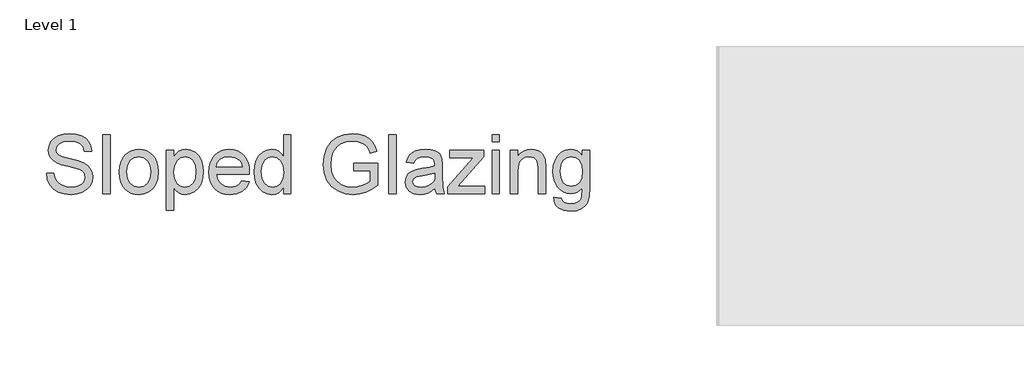
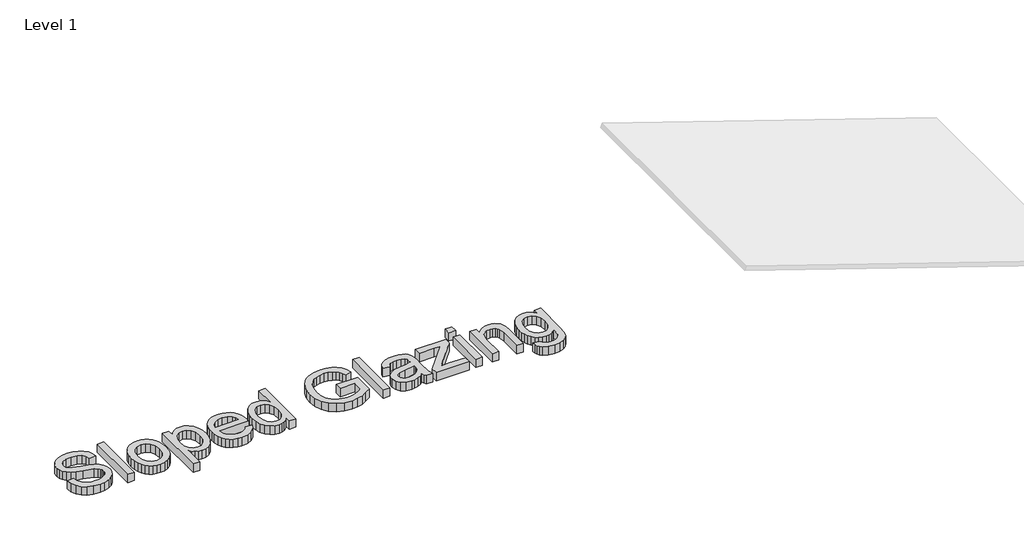
# One storey, part 2 of 42: 1 proxy.
"""IFC4 building model written with IfcOpenShell, lengths in millimetres."""

from ifc_helpers import new_model, si_unit, origin, origin_with_axes, place, context, project, spatial, polyline, outline, extrude, element, save

model = new_model("IFC4")

# Units and contexts
model_context = context("Model", 3, world=origin())
ifc_project = project(units=[si_unit("LENGTHUNIT", "METRE", prefix="MILLI")], contexts=[model_context])

# Site, building, storey
site = spatial("IfcSite", under=ifc_project)
building = spatial("IfcBuilding", under=site)
storey = spatial("IfcBuildingStorey", under=building, Name="Level 1", Elevation=0.0)

# Proxy
placement = place(None, origin())
element("IfcBuildingElementProxy", 1, Name="8\" Arial", ObjectType="8\" Arial", at=placement, inside=storey, context=model_context, shape_type="SweptSolid", body=[
    extrude(outline(polyline([(-16238.469704, -17307.7453742), (-16200.3988172, -17307.7453742), (-16196.0303317, -17328.8721139), (-16188.1298791, -17345.8534396), (-16175.8051731, -17359.3306822), (-16158.1639273, -17369.9451726), (-16136.600339, -17376.8325083), (-16112.508606, -17379.1282869), (-16091.2982145, -17377.3901873), (-16072.7275036, -17372.1758886), (-16057.6794652, -17363.9222394), (-16047.0370908, -17353.0660881), (-16040.7074341, -17340.6019623), (-16038.5975485, -17327.5243896), (-16040.177639, -17314.7814243), (-16044.9179106, -17303.767264), (-16054.5471681, -17294.3703728), (-16070.7942164, -17286.4792148), (-16126.2275095, -17271.9423821), (-16162.6160646, -17262.3224192), (-16185.8991631, -17253.1671889), (-16204.8509546, -17240.3591611), (-16218.281724, -17224.8370954), (-16226.2844177, -17206.9355994), (-16228.9519823, -17186.9892803), (-16225.6523815, -17164.6914147), (-16215.7535792, -17143.8992825), (-16199.5158255, -17126.2766259), (-16177.1993706, -17113.4871874), (-16150.4121891, -17105.7075653), (-16120.7622553, -17103.1143579), (-16088.6399446, -17105.8283957), (-16060.5329227, -17113.9705092), (-16037.4450119, -17127.3733946), (-16020.3800344, -17145.8697483), (-16009.579651, -17168.3070336), (-16005.2855226, -17193.532714), (-16043.3564094, -17193.532714), (-16050.3459862, -17170.8165891), (-16064.9199976, -17154.4208264), (-16087.6918903, -17144.4941401), (-16119.2751113, -17141.1852447), (-16151.6019043, -17144.4569615), (-16173.7789394, -17154.272112), (-16186.6055565, -17168.7159982), (-16190.8810956, -17185.8739223), (-16187.8510396, -17200.5037015), (-16178.7608718, -17212.2707285), (-16157.2716408, -17222.7922724), (-16116.5982521, -17233.5368879), (-16074.6236123, -17243.7424137), (-16049.2306282, -17252.6466885), (-16027.5276203, -17266.4585385), (-16012.3866353, -17283.5049268), (-16003.4916551, -17303.5999603), (-16000.5266618, -17326.557746), (-16003.9377983, -17350.0267375), (-16014.1712081, -17372.1015314), (-16030.8086318, -17391.0997962), (-16053.4318101, -17405.3392001), (-16080.6372509, -17414.2341803), (-16111.021462, -17417.1991737), (-16148.3208928, -17414.001814), (-16179.021122, -17404.4097351), (-16203.4753464, -17388.3857584), (-16222.0367627, -17365.8927052), (-16233.9525041, -17338.4920767), (-16238.469704, -17307.7453742)])), origin_with_axes(), (0.0, 0.0, 1.0), 50.8),
    extrude(outline(polyline([(-15948.1791925, -17412.4403128), (-15948.1791925, -17107.8732187), (-15910.1083057, -17107.8732187), (-15910.1083057, -17412.4403128), (-15948.1791925, -17412.4403128)])), origin_with_axes(), (0.0, 0.0, 1.0), 50.8),
    extrude(outline(polyline([(-15862.5196973, -17300.607083), (-15860.4609323, -17271.640306), (-15854.2846373, -17246.6795232), (-15843.9908123, -17225.7247345), (-15829.5794574, -17208.7759401), (-15815.0705086, -17197.9430254), (-15799.0558265, -17190.2052292), (-15781.5354111, -17185.5625515), (-15762.5092623, -17184.0149923), (-15741.5056768, -17185.8994826), (-15722.514383, -17191.5529535), (-15705.535381, -17200.975405), (-15690.5686706, -17214.1668371), (-15678.3531768, -17230.6811067), (-15669.627824, -17250.0720704), (-15664.3926123, -17272.3397284), (-15662.6475418, -17297.4840805), (-15665.7333656, -17335.9453426), (-15674.9908371, -17365.2234904), (-15690.1504114, -17387.1495699), (-15710.9425436, -17403.5546273), (-15735.6384289, -17413.7880371), (-15762.5092623, -17417.1991737), (-15783.8195713, -17415.3216543), (-15802.9874635, -17409.6890964), (-15820.0129388, -17400.3014998), (-15834.8959972, -17387.1588646), (-15846.981366, -17370.4842623), (-15855.6137723, -17350.5007646), (-15860.793216, -17327.2083715), (-15862.5196973, -17300.607083)]), holes=[polyline([(-15824.4488105, -17300.5327258), (-15820.0431464, -17334.9879936), (-15806.8261539, -17359.5351645), (-15786.9356028, -17374.2300063), (-15762.5092623, -17379.1282869), (-15738.1944577, -17374.2021224), (-15718.3410851, -17359.4236287), (-15705.1240927, -17334.5511451), (-15700.7184285, -17299.3430105), (-15705.1519766, -17265.8915649), (-15718.4526209, -17241.6790014), (-15738.3338774, -17226.9841596), (-15762.5092623, -17222.085879), (-15786.9356028, -17226.9655703), (-15806.8261539, -17241.6046442), (-15820.0431464, -17266.0960472), (-15824.4488105, -17300.5327258)])]), origin_with_axes(), (0.0, 0.0, 1.0), 50.8),
    extrude(outline(polyline([(-15619.8177942, -17498.099808), (-15619.8177942, -17188.7738531), (-15581.7469074, -17188.7738531), (-15581.7469074, -17226.1011679), (-15569.3292549, -17207.688466), (-15555.4244584, -17194.5365362), (-15539.2145886, -17186.6453782), (-15519.8817164, -17184.0149923), (-15494.1355357, -17187.6956737), (-15471.6238932, -17198.737718), (-15453.2948432, -17216.4719104), (-15440.0964401, -17240.229036), (-15432.1216303, -17268.28029), (-15429.4633604, -17298.8968673), (-15432.4655324, -17331.4560266), (-15441.4720483, -17360.5761653), (-15456.194774, -17384.7794342), (-15476.3455754, -17402.5879837), (-15499.8145669, -17413.5463762), (-15524.4918629, -17417.1991737), (-15541.993689, -17414.7546807), (-15557.6179958, -17407.4212018), (-15570.9929973, -17396.3512735), (-15581.7469074, -17382.6974325), (-15581.7469074, -17498.099808), (-15619.8177942, -17498.099808)]), holes=[polyline([(-15581.7469074, -17302.3916558), (-15577.6293774, -17336.5216109), (-15565.2767875, -17360.3902723), (-15547.0499786, -17374.4437833), (-15525.3097921, -17379.1282869), (-15503.2164088, -17374.2764796), (-15484.5248675, -17359.7210575), (-15471.7819022, -17334.978699), (-15467.5342471, -17299.5660821), (-15471.6796611, -17265.62202), (-15484.1159029, -17241.4187512), (-15502.3148278, -17226.9190971), (-15523.7482909, -17222.085879), (-15545.2654058, -17227.2258205), (-15564.1614295, -17242.645645), (-15577.3505379, -17267.8620307), (-15581.7469074, -17302.3916558)])]), origin_with_axes(), (0.0, 0.0, 1.0), 50.8),
    extrude(outline(polyline([(-15230.0373481, -17345.816261), (-15192.7100334, -17350.5751218), (-15206.159392, -17378.700733), (-15227.6207391, -17399.7252315), (-15256.6107527, -17412.8306881), (-15292.6461111, -17417.1991737), (-15316.2684643, -17415.3146834), (-15337.3161994, -17409.6612124), (-15355.7893165, -17400.2387609), (-15371.6878154, -17387.0473288), (-15384.4726066, -17370.4540547), (-15393.6046004, -17350.8260774), (-15399.0837966, -17328.1633968), (-15400.9101953, -17302.466013), (-15399.0652073, -17275.8972557), (-15393.5302431, -17252.4793848), (-15384.3053029, -17232.2124003), (-15371.3903866, -17215.0963022), (-15355.5337136, -17201.4982291), (-15337.4835031, -17191.7853197), (-15317.2397552, -17185.9575741), (-15294.8024699, -17184.0149923), (-15273.0878437, -17185.9529268), (-15253.4505717, -17191.7667304), (-15235.890654, -17201.4564032), (-15220.4080906, -17215.021945), (-15207.7696902, -17232.1008645), (-15198.7422613, -17252.3306704), (-15193.3258039, -17275.7113627), (-15191.5203181, -17302.2429414), (-15191.7433897, -17312.5042351), (-15362.8393086, -17312.5042351), (-15356.2494016, -17341.0016322), (-15340.941113, -17361.9517735), (-15318.8477297, -17374.8341586), (-15291.9025391, -17379.1282869), (-15271.6402019, -17377.1392318), (-15254.5752243, -17371.1720664), (-15240.7076064, -17360.8550048), (-15230.0373481, -17345.816261)]), holes=[polyline([(-15362.8393086, -17274.4333483), (-15229.5912049, -17274.4333483), (-15234.7404411, -17254.3197255), (-15244.834431, -17239.9316072), (-15267.0300555, -17226.5473111), (-15294.9511843, -17222.085879), (-15320.6137132, -17225.64573), (-15341.8333994, -17236.325283), (-15356.5840091, -17252.9720013), (-15362.8393086, -17274.4333483)])]), origin_with_axes(), (0.0, 0.0, 1.0), 50.8),
    extrude(outline(polyline([(-15015.4424669, -17412.4403128), (-15015.4424669, -17376.5257849), (-15026.8330606, -17394.3203925), (-15040.6309686, -17407.0308265), (-15056.8361911, -17414.6570869), (-15075.4487279, -17417.1991737), (-15100.0609613, -17413.5184922), (-15122.5911931, -17402.4764479), (-15141.6638151, -17384.8444967), (-15155.903219, -17361.3940945), (-15164.7703152, -17333.0732957), (-15167.7260139, -17300.8301546), (-15165.0026814, -17268.9866834), (-15156.832684, -17240.229036), (-15143.2253163, -17216.1930709), (-15124.1898729, -17198.5146464), (-15101.1670246, -17187.6399058), (-15075.5974423, -17184.0149923), (-15056.9709635, -17186.6081996), (-15040.5008435, -17194.3878218), (-15026.5402791, -17206.3128578), (-15015.4424669, -17221.342307), (-15015.4424669, -17107.8732187), (-14977.3715801, -17107.8732187), (-14977.3715801, -17412.4403128), (-15015.4424669, -17412.4403128)]), holes=[polyline([(-15129.6551272, -17300.6814402), (-15125.3609988, -17335.1181187), (-15112.4786138, -17359.6095217), (-15093.7591885, -17374.2485956), (-15071.9539394, -17379.1282869), (-15050.157985, -17374.4716672), (-15031.9125868, -17360.5018081), (-15019.5599969, -17336.9584595), (-15015.4424669, -17303.581371), (-15019.6343541, -17267.0905747), (-15032.2100156, -17241.7905372), (-15050.9201463, -17227.0120436), (-15073.5154406, -17222.085879), (-15095.5437613, -17226.8168559), (-15113.5939718, -17241.0097866), (-15125.6398383, -17265.3896538), (-15129.6551272, -17300.6814402)])]), origin_with_axes(), (0.0, 0.0, 1.0), 50.8),
    extrude(outline(polyline([(-14653.7690427, -17293.4687917), (-14653.7690427, -17255.3979049), (-14530.0386607, -17255.3979049), (-14530.0386607, -17369.2387792), (-14560.1068538, -17390.1517419), (-14591.1231011, -17405.1533071), (-14623.0130455, -17414.187707), (-14655.7023299, -17417.1991737), (-14698.4112471, -17412.4124289), (-14737.0119289, -17398.0521945), (-14769.0784717, -17374.6203816), (-14792.1849718, -17342.6189014), (-14806.1548309, -17304.2319965), (-14810.8114506, -17261.6439098), (-14806.1734202, -17218.7490996), (-14792.259329, -17178.8471668), (-14769.6454453, -17145.3771318), (-14755.2921819, -17132.3437088), (-14738.9080375, -17121.7780153), (-14701.4691869, -17107.7802722), (-14658.7509751, -17103.1143579), (-14627.3908257, -17105.8191011), (-14599.1908574, -17113.9333306), (-14575.4430264, -17126.8714835), (-14557.4392892, -17144.0479969), (-14544.1200556, -17166.2900945), (-14534.4257356, -17194.4250004), (-14569.5223343, -17204.3145081), (-14577.3577243, -17184.2473585), (-14586.8847407, -17169.1063735), (-14599.4882862, -17157.6925432), (-14616.5532637, -17148.8068577), (-14636.8992528, -17143.0906479), (-14659.3458327, -17141.1852447), (-14685.6218085, -17143.2393623), (-14708.0869778, -17149.4017153), (-14726.6576887, -17158.9008477), (-14741.2502893, -17170.9653035), (-14760.8434117, -17200.2992192), (-14769.7662758, -17229.0382773), (-14772.7405638, -17260.0824086), (-14769.1621235, -17296.489553), (-14758.4268027, -17326.4462102), (-14740.859914, -17349.7386033), (-14716.7867703, -17366.1529554), (-14688.6146859, -17375.884454), (-14658.7509751, -17379.1282869), (-14632.3820528, -17376.6837939), (-14606.663756, -17369.350315), (-14584.3287119, -17359.2470304), (-14568.1095475, -17348.4931202), (-14568.1095475, -17293.4687917), (-14653.7690427, -17293.4687917)])), origin_with_axes(), (0.0, 0.0, 1.0), 50.8),
    extrude(outline(polyline([(-14472.9323306, -17412.4403128), (-14472.9323306, -17107.8732187), (-14434.8614438, -17107.8732187), (-14434.8614438, -17412.4403128), (-14472.9323306, -17412.4403128)])), origin_with_axes(), (0.0, 0.0, 1.0), 50.8),
    extrude(outline(polyline([(-14234.9892883, -17383.8871477), (-14253.1789186, -17399.4835706), (-14271.9076385, -17409.6890964), (-14291.603002, -17415.3216543), (-14312.6925631, -17417.1991737), (-14344.5081503, -17412.6819737), (-14367.9771418, -17399.1303739), (-14382.448912, -17378.5520186), (-14387.2728354, -17352.9545523), (-14385.451084, -17337.1722364), (-14379.9858297, -17322.839886), (-14371.5555821, -17310.5709479), (-14360.8388505, -17300.978869), (-14334.1817941, -17288.4868592), (-14301.2415542, -17282.7613548), (-14262.3155596, -17276.7384215), (-14235.2123599, -17269.6744875), (-14234.9892883, -17261.1977666), (-14237.6103797, -17244.2071462), (-14245.4736536, -17233.0907447), (-14263.0591316, -17224.8370954), (-14287.5598292, -17222.085879), (-14310.2387754, -17223.9169251), (-14326.0768592, -17229.4100633), (-14336.8772426, -17239.5691158), (-14344.4430878, -17255.3979049), (-14382.5139745, -17250.6390441), (-14375.9054783, -17229.8190279), (-14366.0438546, -17213.4604437), (-14352.0089329, -17200.9498447), (-14332.8805431, -17191.6737839), (-14309.4859088, -17185.9296902), (-14282.652254, -17184.0149923), (-14256.9153679, -17185.7066186), (-14236.513611, -17190.7814975), (-14221.1309651, -17198.4124052), (-14210.4514121, -17207.7721179), (-14203.3688887, -17219.3439572), (-14198.7773316, -17233.6112451), (-14196.9184016, -17266.923271), (-14196.9184016, -17314.2888079), (-14194.9851144, -17380.4295379), (-14187.4006799, -17412.4403128), (-14225.4715666, -17412.4403128), (-14231.5688571, -17399.2047311), (-14234.9892883, -17383.8871477)]), holes=[polyline([(-14234.9892883, -17307.7453742), (-14296.4083361, -17319.4194547), (-14329.162683, -17325.5911024), (-14343.9969446, -17335.6293245), (-14349.2019486, -17350.277693), (-14346.3670803, -17361.5985768), (-14337.8624755, -17370.8746376), (-14323.8740271, -17377.0648746), (-14304.5876282, -17379.1282869), (-14284.139398, -17376.8510976), (-14266.0705982, -17370.0195298), (-14251.4222297, -17359.9534238), (-14241.2352932, -17347.9726198), (-14236.7180933, -17335.6293245), (-14235.2123599, -17318.5271683), (-14234.9892883, -17307.7453742)])]), origin_with_axes(), (0.0, 0.0, 1.0), 50.8),
    extrude(outline(polyline([(-14168.3652365, -17412.4403128), (-14168.3652365, -17376.6001421), (-14036.9760629, -17226.8447399), (-14075.8648788, -17226.8447399), (-14158.8475148, -17226.8447399), (-14158.8475148, -17188.7738531), (-13982.7696636, -17188.7738531), (-13982.7696636, -17221.1192354), (-14099.2873971, -17353.9955531), (-14117.1331252, -17374.3694261), (-14073.1136624, -17374.3694261), (-13978.0108027, -17374.3694261), (-13978.0108027, -17412.4403128), (-14168.3652365, -17412.4403128)])), origin_with_axes(), (0.0, 0.0, 1.0), 50.8),
    extrude(outline(polyline([(-13939.939916, -17412.4403128), (-13939.939916, -17188.7738531), (-13901.8690292, -17188.7738531), (-13901.8690292, -17412.4403128), (-13939.939916, -17412.4403128)])), origin_with_axes(), (0.0, 0.0, 1.0), 50.8),
    extrude(outline(polyline([(-13939.939916, -17145.9441055), (-13939.939916, -17107.8732187), (-13901.8690292, -17107.8732187), (-13901.8690292, -17145.9441055), (-13939.939916, -17145.9441055)])), origin_with_axes(), (0.0, 0.0, 1.0), 50.8),
    extrude(outline(polyline([(-13844.7626991, -17412.4403128), (-13844.7626991, -17188.7738531), (-13806.6918123, -17188.7738531), (-13806.6918123, -17220.0038774), (-13793.4655252, -17204.2587402), (-13777.5809682, -17193.0122135), (-13759.0381413, -17186.2642976), (-13737.8370445, -17184.0149923), (-13719.0711459, -17185.827449), (-13701.8853379, -17191.2648193), (-13687.5529875, -17199.6485937), (-13677.3474617, -17210.3002627), (-13665.9336314, -17238.2957488), (-13663.925987, -17275.1025631), (-13663.925987, -17412.4403128), (-13701.9968737, -17412.4403128), (-13701.9968737, -17280.23321), (-13706.3839486, -17246.5493981), (-13712.4533551, -17236.5204706), (-13721.8874249, -17228.7408485), (-13733.9797647, -17223.7496214), (-13748.023981, -17222.085879), (-13770.3218465, -17225.8223284), (-13789.3294059, -17237.0316764), (-13796.9254587, -17246.1822594), (-13802.3512107, -17258.6882111), (-13806.6918123, -17293.7662205), (-13806.6918123, -17412.4403128), (-13844.7626991, -17412.4403128)])), origin_with_axes(), (0.0, 0.0, 1.0), 50.8),
    extrude(outline(polyline([(-13621.0962394, -17431.4757562), (-13583.0253526, -17436.234617), (-13578.8241708, -17448.1317691), (-13570.6820573, -17456.3110612), (-13554.6766698, -17462.6686019), (-13533.7265285, -17464.7877821), (-13511.3821897, -17462.3897624), (-13494.7633554, -17455.1957032), (-13483.2379893, -17443.6703371), (-13476.1740552, -17428.2783966), (-13473.5715532, -17383.8871477), (-13486.2401612, -17396.3791575), (-13500.377324, -17405.3020215), (-13515.9830415, -17410.65574), (-13533.0573137, -17412.4403128), (-13553.9307742, -17410.3629585), (-13572.308621, -17404.1308956), (-13588.1908544, -17393.7441242), (-13601.5774742, -17379.2026441), (-13612.1989356, -17361.7565859), (-13619.7856937, -17342.65608), (-13624.3377486, -17321.9011263), (-13625.8551002, -17299.4917249), (-13623.1317677, -17268.7543171), (-13614.9617703, -17240.4892862), (-13601.6332421, -17216.5369729), (-13583.4343172, -17198.737718), (-13560.9877372, -17187.6956737), (-13534.9162437, -17184.0149923), (-13517.1123415, -17186.0969939), (-13500.9535923, -17192.3429987), (-13486.4399962, -17202.7530068), (-13473.5715532, -17217.3270182), (-13473.5715532, -17188.7738531), (-13435.5006664, -17188.7738531), (-13435.5006664, -17381.8795033), (-13438.1031684, -17426.4659398), (-13445.9106745, -17455.8277394), (-13459.3600332, -17475.3000314), (-13478.888093, -17490.2179447), (-13504.0673001, -17499.6984878), (-13534.4701005, -17502.8586689), (-13569.892012, -17498.4065315), (-13597.7852569, -17485.0501193), (-13608.2905352, -17475.0235155), (-13615.6774584, -17462.7522537), (-13619.9460264, -17448.236334), (-13621.0962394, -17431.4757562)]), holes=[polyline([(-13587.7842134, -17296.8892229), (-13583.7224514, -17331.8092233), (-13571.5371651, -17355.8173045), (-13553.2174098, -17369.7313957), (-13530.7522405, -17374.3694261), (-13508.4543749, -17369.7592796), (-13490.0416731, -17355.9288403), (-13477.6890832, -17332.2274826), (-13473.5715532, -17298.0045809), (-13477.8099136, -17264.9992785), (-13490.5249949, -17241.2328582), (-13509.2072416, -17226.8726238), (-13531.3470981, -17222.085879), (-13553.0872847, -17226.7982666), (-13571.3140935, -17240.9354294), (-13583.6666835, -17264.348653), (-13587.7842134, -17296.8892229)])]), origin_with_axes(), (0.0, 0.0, 1.0), 50.8),
])

save(model, "model.ifc")

# Revit data of these elements
# Element 1 (IfcBuildingElementProxy, "8\" Arial")
#   Phase Created = New Construction
